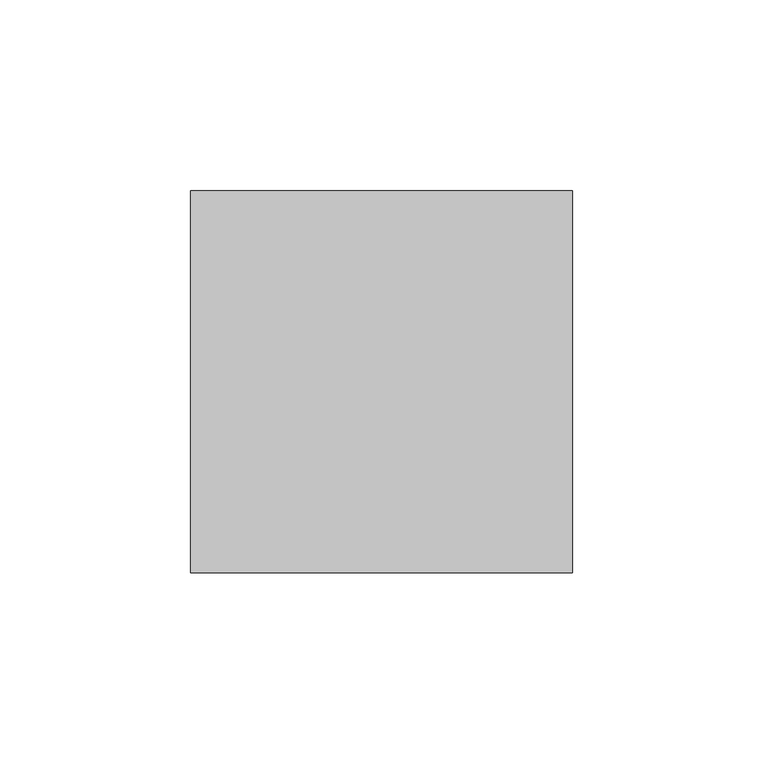
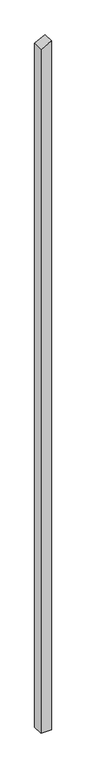
"""IFC4 building model written with IfcOpenShell, lengths in millimetres: column geometry, Holzstütze 159956 : Holzstütze 159956."""

from ifc_helpers import new_model, si_unit, frame, origin, place, context, project, spatial, polyline, outline, extrude, source, transform, mapped, element, save


def column_527da152(model_context):
    return source(origin(), model_context, "Body", "SweptSolid", [
        extrude(outline(polyline([(-500.0, 157297.7593015), (-500.0, 157397.7593015), (6396.6643707, 157397.7593015), (6345.7118258, 157297.7593015), (-500.0, 157297.7593015)])), frame((0.0, 35528.3551606, 0.0), z_axis=(0.0, 1.0, 0.0), x_axis=(0.0, 0.0, 1.0)), (0.0, 0.0, 1.0), 100.0),
    ])


if __name__ == "__main__":
    model = new_model("IFC4")
    model_context = context("Model", 3, world=origin())
    ifc_project = project(units=[si_unit("LENGTHUNIT", "METRE", prefix="MILLI")], contexts=[model_context])
    site = spatial("IfcSite", under=ifc_project)
    building = spatial("IfcBuilding", under=site)
    placement = place(None, origin())
    column_shape = column_527da152(model_context)
    element("IfcColumn", 1, ObjectType="Holzstütze 159956 : Holzstütze 159956", at=placement, inside=building, context=model_context, shape_type="MappedRepresentation", body=[
        mapped(column_shape, transform((0.0, 0.0, 0.0), x_axis=(1.0, 0.0, 0.0), y_axis=(0.0, 1.0, 0.0), z_axis=(0.0, 0.0, 1.0))),
    ])
    save(model, "model.ifc")

# Revit data of these elements
# Type "Holzstütze 159956 : Holzstütze 159956"
#   Abrechnungsart = "m"
#   Allright_Bauteil_ID = "0152St 0000143346"
#   Bezeichnung = "Holzstütze"
#   Codetext = "ST-HOLZ\\"
#   Gewerk = "Zimmer- und Holzbauarbeiten"
#   Material = "Holz"
#   Objektname = "Stütze"
#   NameOverride = "Holzstütze"
#   Reference = "Holzstütze"
#   Status = "NEW"
#   ThermalTransmittance = 0.0000 BTU/(h·ft²·°F)
#   Roll = 0.00°
#   Slope = 0.00°
#   2D Interaktion = yes
#   IsExternal = yes
#   LoadBearing = yes
# Element 1 (IfcColumn, "Holzstütze 159956 : Holzstütze 159956")
#   Materials on its faces: "holzschalung"
# Materials
#   "holzschalung": class "Unassigned", colour RGB 128 128 128, transparency 0
